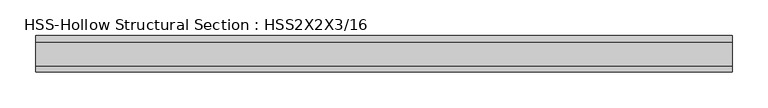
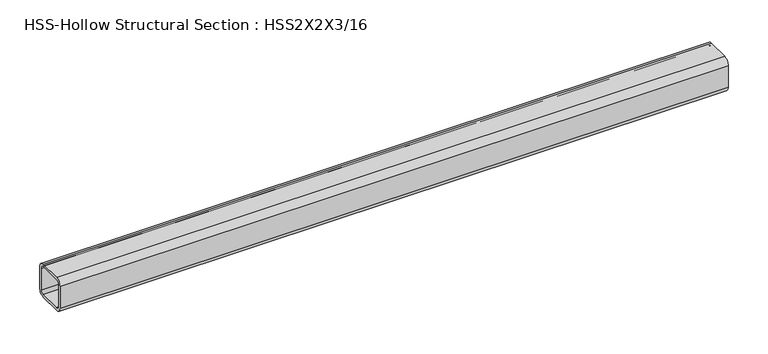
"""IFC4 building model written with IfcOpenShell, lengths in millimetres: beam geometry, HSS-Hollow Structural Section : HSS2X2X3/16."""

from ifc_helpers import new_model, si_unit, point, frame, frame_2d, origin, place, context, project, spatial, polyline, circle_curve, trimmed, segment, composite_curve, outline, extrude, source, transform, mapped, element, save


def hss_hollow_structural_section_hss2x2x3_16_abbce518(model_context):
    return source(origin(), model_context, "Body", "SweptSolid", [
        extrude(outline(composite_curve([segment(polyline([(25.4, 16.5608), (25.4, -16.5608)]), True, "CONTINUOUS"), segment(trimmed(circle_curve(frame_2d((16.5608, -16.5608)), 8.8392), [point((25.4, -16.5608))], [point((16.5608, -25.4))], False, "CARTESIAN"), True, "CONTINUOUS"), segment(polyline([(16.5608, -25.4), (-16.5608, -25.4)]), True, "CONTINUOUS"), segment(trimmed(circle_curve(frame_2d((-16.5608, -16.5608)), 8.8392), [point((-16.5608, -25.4))], [point((-25.4, -16.5608))], False, "CARTESIAN"), True, "CONTINUOUS"), segment(polyline([(-25.4, -16.5608), (-25.4, 16.5608)]), True, "CONTINUOUS"), segment(trimmed(circle_curve(frame_2d((-16.5608, 16.5608)), 8.8392), [point((-25.4, 16.5608))], [point((-16.5608, 25.4))], False, "CARTESIAN"), True, "CONTINUOUS"), segment(polyline([(-16.5608, 25.4), (16.5608, 25.4)]), True, "CONTINUOUS"), segment(trimmed(circle_curve(frame_2d((16.5608, 16.5608)), 8.8392), [point((16.5608, 25.4))], [point((25.4, 16.5608))], False, "CARTESIAN"), True, "CONTINUOUS")], self_intersect=False), holes=[composite_curve([segment(trimmed(circle_curve(frame_2d((-16.5608, 16.5608)), 4.4196), [point((-16.5608, 20.9804))], [point((-20.9804, 16.5608))], True, "CARTESIAN"), True, "CONTINUOUS"), segment(polyline([(-20.9804, 16.5608), (-20.9804, -16.5608)]), True, "CONTINUOUS"), segment(trimmed(circle_curve(frame_2d((-16.5608, -16.5608)), 4.4196), [point((-20.9804, -16.5608))], [point((-16.5608, -20.9804))], True, "CARTESIAN"), True, "CONTINUOUS"), segment(polyline([(-16.5608, -20.9804), (16.5608, -20.9804)]), True, "CONTINUOUS"), segment(trimmed(circle_curve(frame_2d((16.5608, -16.5608)), 4.4196), [point((16.5608, -20.9804))], [point((20.9804, -16.5608))], True, "CARTESIAN"), True, "CONTINUOUS"), segment(polyline([(20.9804, -16.5608), (20.9804, 16.5608)]), True, "CONTINUOUS"), segment(trimmed(circle_curve(frame_2d((16.5608, 16.5608)), 4.4196), [point((20.9804, 16.5608))], [point((16.5608, 20.9804))], True, "CARTESIAN"), True, "CONTINUOUS"), segment(polyline([(16.5608, 20.9804), (-16.5608, 20.9804)]), True, "CONTINUOUS")], self_intersect=False)]), frame((-863.6, 0.0, 0.0), z_axis=(1.0, 0.0, 0.0), x_axis=(0.0, 1.0, 0.0)), (0.0, 0.0, 1.0), 968.375),
    ])


if __name__ == "__main__":
    model = new_model("IFC4")
    model_context = context("Model", 3, world=origin())
    ifc_project = project(units=[si_unit("LENGTHUNIT", "METRE", prefix="MILLI")], contexts=[model_context])
    site = spatial("IfcSite", under=ifc_project)
    building = spatial("IfcBuilding", under=site)
    placement = place(None, origin())
    hss_hollow_structural_section_hss2x2x3_16_shape = hss_hollow_structural_section_hss2x2x3_16_abbce518(model_context)
    element("IfcBeam", 1, ObjectType="HSS-Hollow Structural Section : HSS2X2X3/16", at=placement, inside=building, context=model_context, shape_type="MappedRepresentation", body=[
        mapped(hss_hollow_structural_section_hss2x2x3_16_shape, transform((0.0, 0.0, 0.0), x_axis=(1.0, 0.0, 0.0), y_axis=(0.0, 1.0, 0.0), z_axis=(0.0, 0.0, 1.0))),
    ])
    save(model, "model.ifc")

# Revit data of these elements
# Type "HSS-Hollow Structural Section : HSS2X2X3/16"
#   Keynote = "M05121300.04"
#   Assembly Code = "B10"
#   Shape = "Square"
#   W = 4.3
#   Ht = 0' - 2"
#   Length [instance default] = 5' - 0"
#   b = 0' - 2"
#   kr = 0' - 0.348"
#   t = 0' - 0.174"
#   A = 0.00826389 SF
#   Structural Material [instance default] = Steel ASTM A500, Grade B, Rectangular and Square
# Element 1 (IfcBeam, "HSS-Hollow Structural Section : HSS2X2X3/16")
#   Structural Material = none
# Materials
#   "Steel ASTM A500, Grade B, Rectangular and Square": class "Metal", colour RGB 199 199 199, transparency 0, Description = "Carbon steel", Cost = 0
